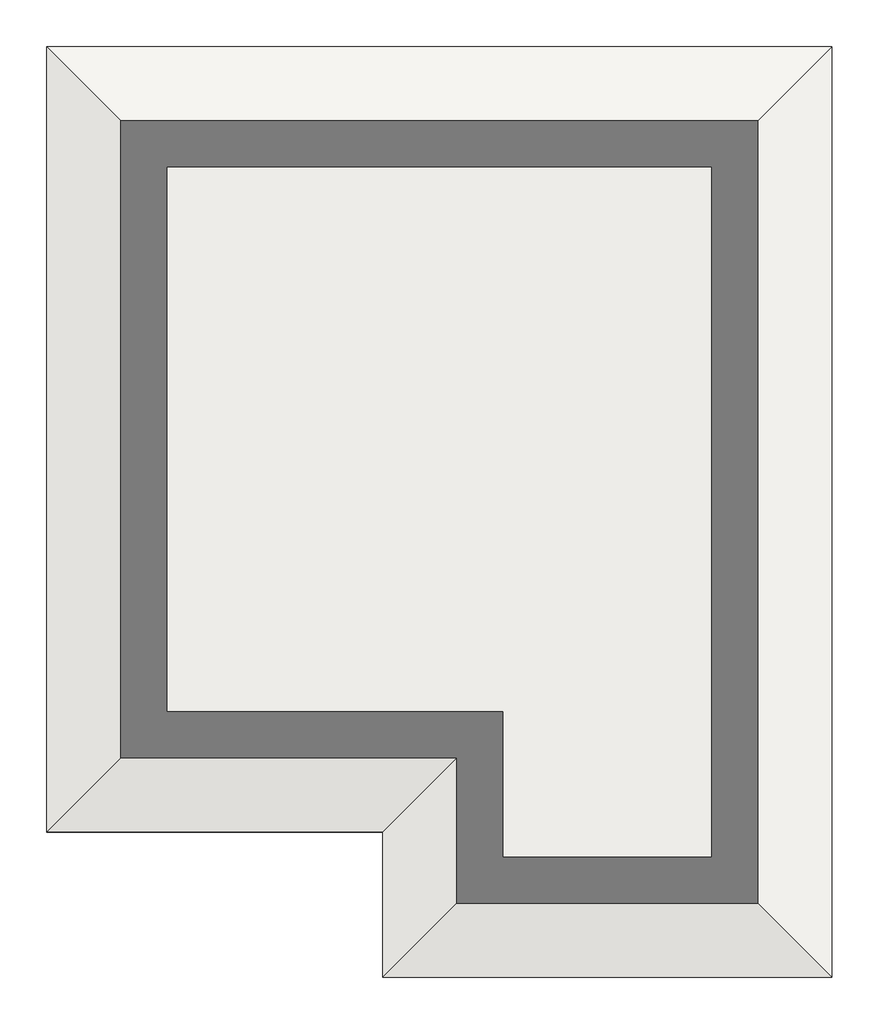
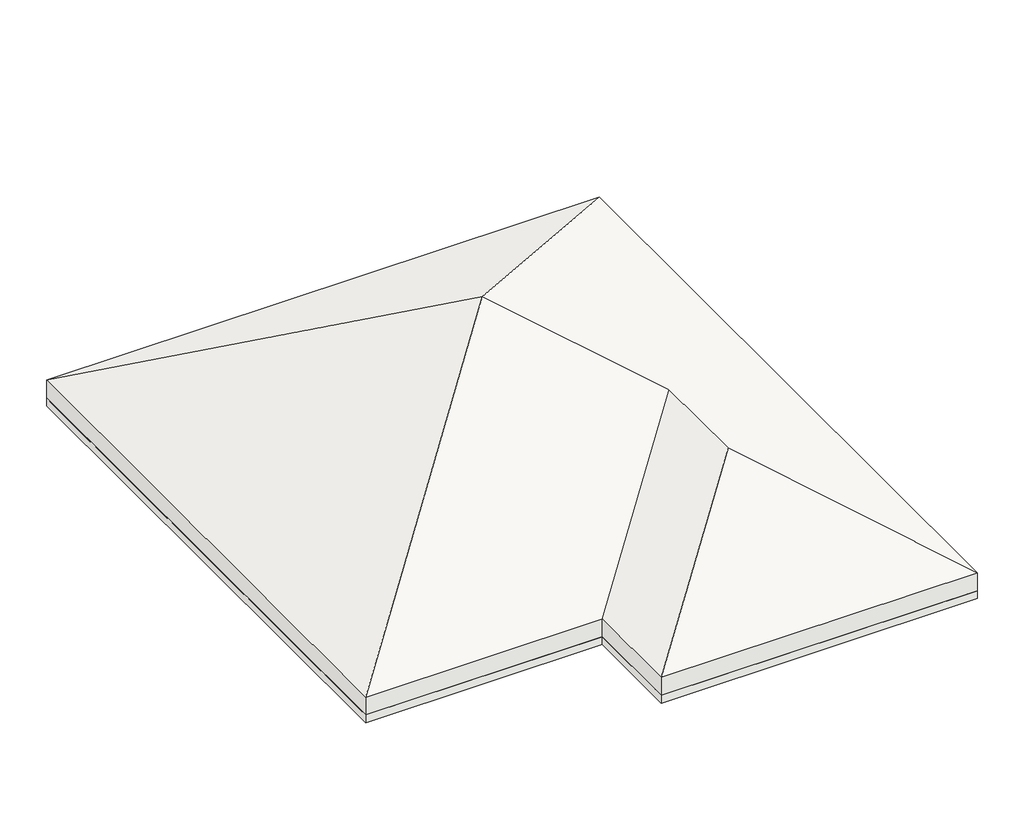
# One storey: 15 beams, 6 walls, 1 roof, 1 slab.
"""IFC4 building model written with IfcOpenShell, lengths in millimetres."""

import ifcopenshell
import ifcopenshell.guid

model = None  # the IFC model being written
_history = None  # IfcOwnerHistory: only IFC2X3 demands one
_inside = {}  # id of a spatial element -> (the spatial element, [elements in it])
_under = {}  # id of a project, library or spatial element -> (it, [spatial elements below it])
_declared = {}  # id of a project -> (the project, [libraries it declares])
_typed = {}  # id of a type object -> (the type object, [elements of that type])
_made_of = {}  # id of a material, layer set ... -> (it, [elements and type objects made of it])


def new_model(schema):
    """Start an empty IFC model of exactly this schema.

    Asked for "IFC4X3", IfcOpenShell would pick the latest addendum, in which some entities
    have other attributes; the version numbers below select the first issue.
    IFC2X3 requires an IfcOwnerHistory on every rooted entity: one is made here for all.
    """
    global model, _history
    if schema == "IFC4X3":
        model = ifcopenshell.file(schema_version=(4, 3, 0, 0))
    else:
        model = ifcopenshell.file(schema=schema)
    _inside.clear()
    _under.clear()
    _declared.clear()
    _typed.clear()
    _made_of.clear()
    _history = None
    if model.schema == "IFC2X3":
        org = make("IfcOrganization", Name="unknown")
        user = make(
            "IfcPersonAndOrganization",
            ThePerson=make("IfcPerson", FamilyName="unknown"),
            TheOrganization=org,
        )
        app = make(
            "IfcApplication",
            ApplicationDeveloper=org,
            Version="unknown",
            ApplicationFullName="unknown",
            ApplicationIdentifier="unknown",
        )
        _history = make(
            "IfcOwnerHistory",
            OwningUser=user,
            OwningApplication=app,
            ChangeAction="ADDED",
            CreationDate=0,
        )
    return model


def make(cls, **values):
    """One entity of the class cls with the attributes given. An attribute that is None is left unset."""
    return model.create_entity(
        cls, **{name: value for name, value in values.items() if value is not None}
    )


def rooted(cls, **values):
    """An entity with a GlobalId (a new one), such as an element, a storey or a relation."""
    return make(cls, GlobalId=ifcopenshell.guid.new(), OwnerHistory=_history, **values)


def si_unit(unit_type, name, prefix=None):
    """IfcSIUnit, for example si_unit("LENGTHUNIT", "METRE", prefix="MILLI")."""
    return make("IfcSIUnit", UnitType=unit_type, Prefix=prefix, Name=name)


def assignment(units):
    """IfcUnitAssignment: the units of a project."""
    return None if units is None else make("IfcUnitAssignment", Units=units)


def point(xyz):
    """IfcCartesianPoint."""
    return None if xyz is None else make("IfcCartesianPoint", Coordinates=xyz)


def direction(xyz):
    """IfcDirection."""
    return None if xyz is None else make("IfcDirection", DirectionRatios=xyz)


def frame(location, z_axis=None, x_axis=None):
    """IfcAxis2Placement3D, a coordinate frame: its origin and axes. An axis left out is left unset."""
    return make(
        "IfcAxis2Placement3D",
        Location=point(location),
        Axis=direction(z_axis),
        RefDirection=direction(x_axis),
    )


def origin():
    """The frame at (0, 0, 0) with its axes left unset."""
    return frame((0.0, 0.0, 0.0))


def place(relative_to, where):
    """IfcLocalPlacement: puts the frame where relative to a parent placement (None: the world)."""
    return make(
        "IfcLocalPlacement", PlacementRelTo=relative_to, RelativePlacement=where
    )


def context(
    kind, dimensions, precision=None, world=None, true_north=None, identifier=None
):
    """IfcGeometricRepresentationContext, for example the 3D "Model" context."""
    return make(
        "IfcGeometricRepresentationContext",
        ContextIdentifier=identifier,
        ContextType=kind,
        CoordinateSpaceDimension=dimensions,
        Precision=precision,
        WorldCoordinateSystem=world,
        TrueNorth=true_north,
    )


def project(units=None, contexts=None):
    """IfcProject with its units and contexts."""
    return rooted(
        "IfcProject",
        Name="project",
        RepresentationContexts=contexts,
        UnitsInContext=assignment(units),
    )


def spatial(cls, under=None, at=None, **own):
    """A site, building, storey or space (cls), placed at a placement, below another one or the project."""
    s = rooted(cls, ObjectPlacement=at, **own)
    if under is not None:
        _under.setdefault(under.id(), (under, []))[1].append(s)
    return s


def polyline(points):
    """IfcPolyline through the points."""
    return make("IfcPolyline", Points=[point(p) for p in points])


def outline(outer, holes=None, kind="AREA"):
    """IfcArbitraryClosedProfileDef: a profile drawn as a closed curve; with holes, ...WithVoids."""
    if holes is None:
        return make("IfcArbitraryClosedProfileDef", ProfileType=kind, OuterCurve=outer)
    return make(
        "IfcArbitraryProfileDefWithVoids",
        ProfileType=kind,
        OuterCurve=outer,
        InnerCurves=holes,
    )


def extrude(swept, where, along, depth):
    """IfcExtrudedAreaSolid: the profile swept, set in the frame where, extruded along a direction by depth."""
    return make(
        "IfcExtrudedAreaSolid",
        SweptArea=swept,
        Position=where,
        ExtrudedDirection=direction(along),
        Depth=depth,
    )


def faces_of(points, faces, orient=None, outer=None):
    """IfcFace entities. A face is a list of loops; a loop is a list of indices into points, from 0.

    orient and outer hold one flag for each loop. By default every Orientation is true, the
    first loop of a face is its IfcFaceOuterBound and the others are IfcFaceBound.
    """
    made = []
    for i, loops in enumerate(faces):
        bounds = []
        for j, loop in enumerate(loops):
            is_outer = j == 0 if outer is None else outer[i][j]
            bounds.append(
                make(
                    "IfcFaceOuterBound" if is_outer else "IfcFaceBound",
                    Bound=make("IfcPolyLoop", Polygon=[points[k] for k in loop]),
                    Orientation=True if orient is None else orient[i][j],
                )
            )
        made.append(make("IfcFace", Bounds=bounds))
    return made


def faceted_brep(points, faces, orient=None, outer=None, voids=None):
    """IfcFacetedBrep: a solid bounded by flat faces; with voids (closed shells), ...WithVoids."""
    shared = [point(p) for p in points]
    hull = make("IfcClosedShell", CfsFaces=faces_of(shared, faces, orient, outer))
    if voids is None:
        return make("IfcFacetedBrep", Outer=hull)
    return make(
        "IfcFacetedBrepWithVoids",
        Outer=hull,
        Voids=[
            make(cls, CfsFaces=faces_of(shared, fs, o, b)) for cls, fs, o, b in voids
        ],
    )


def shape(context_of_items, identifier, shape_type, items):
    """IfcShapeRepresentation: the items that make up one representation, for example the "Body"."""
    return make(
        "IfcShapeRepresentation",
        ContextOfItems=context_of_items,
        RepresentationIdentifier=identifier,
        RepresentationType=shape_type,
        Items=items,
    )


def made_of(thing, what):
    """Note that an element or type object is made of a material, layer set ...; save() writes the relation."""
    if what is not None:
        _made_of.setdefault(what.id(), (what, []))[1].append(thing)
    return thing


def element(
    cls,
    number,
    at=None,
    inside=None,
    cuts=None,
    type_object=None,
    material=None,
    context=None,
    identifier="Body",
    shape_type=None,
    held_by="IfcProductDefinitionShape",
    body=None,
    shapes=None,
    **own,
):
    """One element of the class cls, such as IfcWall. Its Tag is "e" and its number.

    at: its placement. inside: the storey or other place that contains it. cuts: it is an
    opening in that element (IfcRelVoidsElement). A single representation is given by context,
    identifier, shape_type and body (its items); several are given by shapes. held_by: the class
    of the entity that holds the representations. save() writes the other relations.
    """
    e = rooted(cls, Tag="e%d" % number, ObjectPlacement=at, **own)
    if body is not None:
        shapes = [shape(context, identifier, shape_type, body)]
    if shapes is not None:
        e.Representation = make(held_by, Representations=shapes)
    if inside is not None:
        _inside.setdefault(inside.id(), (inside, []))[1].append(e)
    if cuts is not None:
        rooted(
            "IfcRelVoidsElement", RelatingBuildingElement=cuts, RelatedOpeningElement=e
        )
    if type_object is not None:
        _typed.setdefault(type_object.id(), (type_object, []))[1].append(e)
    return made_of(e, material)


def aggregate(whole, parts):
    """IfcRelAggregates: a whole, such as a stair, and the parts it consists of."""
    return rooted("IfcRelAggregates", RelatingObject=whole, RelatedObjects=parts)


def save(model, path):
    """Write the relations noted so far, then the file.

    IfcRelAggregates (storeys below a building ...), IfcRelContainedInSpatialStructure (elements
    in a storey), IfcRelDefinesByType, IfcRelAssociatesMaterial and IfcRelDeclares: one each for
    every whole, place, type object, material and project.
    """
    for whole, parts in _under.values():
        aggregate(whole, parts)
    for where, things in _inside.values():
        rooted(
            "IfcRelContainedInSpatialStructure",
            RelatedElements=things,
            RelatingStructure=where,
        )
    for kind, things in _typed.values():
        rooted("IfcRelDefinesByType", RelatedObjects=things, RelatingType=kind)
    for what, things in _made_of.values():
        rooted("IfcRelAssociatesMaterial", RelatedObjects=things, RelatingMaterial=what)
    for by, libraries in _declared.values():
        rooted("IfcRelDeclares", RelatingContext=by, RelatedDefinitions=libraries)
    model.write(path)


model = new_model("IFC4")

# Units and contexts
model_context = context("Model", 3, world=origin())
ifc_project = project(units=[si_unit("LENGTHUNIT", "METRE", prefix="MILLI")], contexts=[model_context])

# Site, building, storey
site = spatial("IfcSite", under=ifc_project)
building = spatial("IfcBuilding", under=site)
storey = spatial("IfcBuildingStorey", under=building, Name="02-Çatı Katı", Elevation=100780.0)

# Beams
placement = place(None, origin())
element("IfcBeam", 1, ObjectType="M_Concrete-Rectangular Beam : 45x60cm Kiriş", at=placement, inside=storey, context=model_context, shape_type="SweptSolid", body=[
    extrude(outline(polyline([(5700.0, 14550.0), (450.0, 14550.0), (450.0, 15000.0), (5700.0, 15000.0), (5700.0, 14550.0)])), frame((0.0, 0.0, 100180.0), z_axis=(0.0, 0.0, 1.0), x_axis=(1.0, 0.0, 0.0)), (0.0, 0.0, 1.0), 400.0),
])
element("IfcBeam", 2, ObjectType="M_Concrete-Rectangular Beam : 45x60cm Kiriş", at=placement, inside=storey, context=model_context, shape_type="SweptSolid", body=[
    extrude(outline(polyline([(0.0, 3100.0), (0.0, 8200.0), (450.0, 8200.0), (450.0, 3100.0), (0.0, 3100.0)])), frame((0.0, 0.0, 100180.0), z_axis=(0.0, 0.0, 1.0), x_axis=(1.0, 0.0, 0.0)), (0.0, 0.0, 1.0), 400.0),
])
element("IfcBeam", 3, ObjectType="M_Concrete-Rectangular Beam : 45x60cm Kiriş", at=placement, inside=storey, context=model_context, shape_type="SweptSolid", body=[
    extrude(outline(polyline([(5700.0, 2500.0), (450.0, 2500.0), (450.0, 2950.0), (5700.0, 2950.0), (5700.0, 2500.0)])), frame((0.0, 0.0, 100180.0), z_axis=(0.0, 0.0, 1.0), x_axis=(1.0, 0.0, 0.0)), (0.0, 0.0, 1.0), 400.0),
])
element("IfcBeam", 4, ObjectType="M_Concrete-Rectangular Beam : 45x60cm Kiriş", at=placement, inside=storey, context=model_context, shape_type="SweptSolid", body=[
    extrude(outline(polyline([(12050.0, 2500.0), (6300.0, 2500.0), (6300.0, 2950.0), (12050.0, 2950.0), (12050.0, 2500.0)])), frame((0.0, 0.0, 100180.0), z_axis=(0.0, 0.0, 1.0), x_axis=(1.0, 0.0, 0.0)), (0.0, 0.0, 1.0), 400.0),
])
element("IfcBeam", 5, ObjectType="M_Concrete-Rectangular Beam : 45x60cm Kiriş", at=placement, inside=storey, context=model_context, shape_type="SweptSolid", body=[
    extrude(outline(polyline([(12500.0, 8200.0), (12500.0, 3100.0), (12050.0, 3100.0), (12050.0, 8200.0), (12500.0, 8200.0)])), frame((0.0, 0.0, 100180.0), z_axis=(0.0, 0.0, 1.0), x_axis=(1.0, 0.0, 0.0)), (0.0, 0.0, 1.0), 400.0),
])
element("IfcBeam", 6, ObjectType="M_Concrete-Rectangular Beam : 45x60cm Kiriş", at=placement, inside=storey, context=model_context, shape_type="SweptSolid", body=[
    extrude(outline(polyline([(0.0, 8800.0), (0.0, 14400.0), (450.0, 14400.0), (450.0, 8800.0), (0.0, 8800.0)])), frame((0.0, 0.0, 100180.0), z_axis=(0.0, 0.0, 1.0), x_axis=(1.0, 0.0, 0.0)), (0.0, 0.0, 1.0), 400.0),
])
element("IfcBeam", 7, ObjectType="M_Concrete-Rectangular Beam : 45x60cm Kiriş", at=placement, inside=storey, context=model_context, shape_type="SweptSolid", body=[
    extrude(outline(polyline([(5775.0, 8800.0), (5775.0, 14550.0), (6225.0, 14550.0), (6225.0, 8800.0), (5775.0, 8800.0)])), frame((0.0, 0.0, 100180.0), z_axis=(0.0, 0.0, 1.0), x_axis=(1.0, 0.0, 0.0)), (0.0, 0.0, 1.0), 400.0),
])
element("IfcBeam", 8, ObjectType="M_Concrete-Rectangular Beam : 30x60cm Kiriş", at=placement, inside=storey, context=model_context, shape_type="SweptSolid", body=[
    extrude(outline(polyline([(9850.0, 15000.0), (9850.0, 14700.0), (6300.0, 14700.0), (6300.0, 15000.0), (9850.0, 15000.0)])), frame((0.0, 0.0, 100180.0), z_axis=(0.0, 0.0, 1.0), x_axis=(1.0, 0.0, 0.0)), (0.0, 0.0, 1.0), 400.0),
])
element("IfcBeam", 9, ObjectType="M_Concrete-Rectangular Beam : 30x60cm Kiriş", at=placement, inside=storey, context=model_context, shape_type="SweptSolid", body=[
    extrude(outline(polyline([(12200.0, 10850.0), (12500.0, 10850.0), (12500.0, 8800.0), (12200.0, 8800.0), (12200.0, 10850.0)])), frame((0.0, 0.0, 100180.0), z_axis=(0.0, 0.0, 1.0), x_axis=(1.0, 0.0, 0.0)), (0.0, 0.0, 1.0), 400.0),
])
element("IfcBeam", 10, ObjectType="M_Concrete-Rectangular Beam : 45x60cm Kiriş", at=placement, inside=storey, context=model_context, shape_type="SweptSolid", body=[
    extrude(outline(polyline([(5775.0, 2950.0), (5775.0, 8200.0), (6225.0, 8200.0), (6225.0, 2950.0), (5775.0, 2950.0)])), frame((0.0, 0.0, 100180.0), z_axis=(0.0, 0.0, 1.0), x_axis=(1.0, 0.0, 0.0)), (0.0, 0.0, 1.0), 400.0),
])
element("IfcBeam", 11, ObjectType="M_Concrete-Rectangular Beam : 45x60cm Kiriş", at=placement, inside=storey, context=model_context, shape_type="SweptSolid", body=[
    extrude(outline(polyline([(5775.0, 8275.0), (450.0, 8275.0), (450.0, 8725.0), (5775.0, 8725.0), (5775.0, 8275.0)])), frame((0.0, 0.0, 100180.0), z_axis=(0.0, 0.0, 1.0), x_axis=(1.0, 0.0, 0.0)), (0.0, 0.0, 1.0), 400.0),
])
element("IfcBeam", 12, ObjectType="M_Concrete-Rectangular Beam : 45x60cm Kiriş", at=placement, inside=storey, context=model_context, shape_type="SweptSolid", body=[
    extrude(outline(polyline([(12050.0, 8275.0), (6225.0, 8275.0), (6225.0, 8725.0), (12050.0, 8725.0), (12050.0, 8275.0)])), frame((0.0, 0.0, 100180.0), z_axis=(0.0, 0.0, 1.0), x_axis=(1.0, 0.0, 0.0)), (0.0, 0.0, 1.0), 400.0),
])
element("IfcBeam", 13, ObjectType="M_Concrete-Rectangular Beam : 45x60cm Kiriş", at=placement, inside=storey, context=model_context, shape_type="Brep", body=[
    faceted_brep([(5775.0, 2500.0, 100180.0), (5775.0, 400.0, 100180.0), (5775.0, 400.0, 100580.0), (5775.0, 2500.0, 100580.0), (6225.0, 2500.0, 100180.0), (6225.0, 450.0, 100180.0), (6225.0, 0.0, 100180.0), (6175.0, 0.0, 100180.0), (6175.0, 400.0, 100180.0), (6225.0, 2500.0, 100580.0), (6225.0, 450.0, 100580.0), (6225.0, 0.0, 100580.0), (6175.0, 0.0, 100580.0), (6175.0, 400.0, 100580.0)], [[[0, 1, 2, 3]], [[0, 4, 5, 6, 7, 8, 1]], [[6, 5, 4, 9, 10, 11]], [[4, 0, 3, 9]], [[8, 7, 12, 13]], [[1, 8, 13, 2]], [[7, 6, 11, 12]], [[3, 2, 13, 12, 11, 10, 9]]]),
])
element("IfcBeam", 14, ObjectType="M_Concrete-Rectangular Beam : 45x60cm Kiriş", at=placement, inside=storey, context=model_context, shape_type="Brep", body=[
    faceted_brep([(6225.0, 0.0, 100180.0), (12100.0, 0.0, 100180.0), (12100.0, 0.0, 100580.0), (6225.0, 0.0, 100580.0), (6225.0, 450.0, 100180.0), (12050.0, 450.0, 100180.0), (12500.0, 450.0, 100180.0), (12500.0, 400.0, 100180.0), (12100.0, 400.0, 100180.0), (6225.0, 450.0, 100580.0), (12050.0, 450.0, 100580.0), (12500.0, 450.0, 100580.0), (12100.0, 400.0, 100580.0), (12500.0, 400.0, 100580.0)], [[[0, 1, 2, 3]], [[0, 4, 5, 6, 7, 8, 1]], [[6, 5, 4, 9, 10, 11]], [[4, 0, 3, 9]], [[1, 8, 12, 2]], [[8, 7, 13, 12]], [[7, 6, 11, 13]], [[3, 2, 12, 13, 11, 10, 9]]]),
])
element("IfcBeam", 15, ObjectType="M_Concrete-Rectangular Beam : 45x60cm Kiriş", at=placement, inside=storey, context=model_context, shape_type="SweptSolid", body=[
    extrude(outline(polyline([(12050.0, 2500.0), (12500.0, 2500.0), (12500.0, 450.0), (12050.0, 450.0), (12050.0, 2500.0)])), frame((0.0, 0.0, 100180.0), z_axis=(0.0, 0.0, 1.0), x_axis=(1.0, 0.0, 0.0)), (0.0, 0.0, 1.0), 400.0),
])

# Roof
element("IfcRoof", 16, ObjectType="Generic - 400mm", at=placement, inside=storey, context=model_context, shape_type="Brep", body=[
    faceted_brep([(-500.0, 2000.0, 100780.0), (-500.0, 15500.0, 100780.0), (6250.0, 8750.0, 104677.114317), (9137.5, 5862.5, 103010.0154147), (5275.0, 2000.0, 100780.0), (5275.0, -500.0, 100780.0), (9137.5, 3362.5, 103010.0154147), (13000.0, -500.0, 100780.0), (13000.0, 15500.0, 100780.0), (-500.0, 2000.0, 101241.8802154), (6250.0, 8750.0, 105138.9945324), (-500.0, 15500.0, 101241.8802154), (5275.0, 2000.0, 101241.8802154), (9137.5, 5862.5, 103471.8956301), (5275.0, -500.0, 101241.8802154), (13000.0, -500.0, 101241.8802154), (9137.5, 3362.5, 103471.8956301), (13000.0, 15500.0, 101241.8802154)], [[[0, 1, 2]], [[0, 2, 3, 4]], [[5, 6, 7]], [[8, 2, 1]], [[7, 6, 3, 2, 8]], [[5, 4, 3, 6]], [[9, 10, 11]], [[9, 12, 13, 10]], [[14, 15, 16]], [[17, 11, 10]], [[15, 17, 10, 13, 16]], [[12, 14, 16, 13]], [[4, 12, 9, 0]], [[5, 14, 12, 4]], [[7, 15, 14, 5]], [[8, 17, 15, 7]], [[1, 11, 17, 8]], [[0, 9, 11, 1]]]),
])

# Slab
element("IfcSlab", 17, ObjectType="20 cm döşeme", at=placement, inside=storey, context=model_context, shape_type="SweptSolid", body=[
    extrude(outline(polyline([(-500.0, 15500.0), (13000.0, 15500.0), (13000.0, -500.0), (5275.0, -500.0), (5275.0, 2000.0), (-500.0, 2000.0), (-500.0, 15500.0)])), frame((0.0, 0.0, 100580.0), z_axis=(0.0, 0.0, 1.0), x_axis=(1.0, 0.0, 0.0)), (0.0, 0.0, 1.0), 200.0),
])

# Walls
element("IfcWall", 18, ObjectType="25cm Perde Duvar", at=placement, inside=storey, context=model_context, shape_type="Brep", body=[
    faceted_brep([(-500.0, 15250.0, 100780.0), (-250.0, 15250.0, 100780.0), (12750.0, 15250.0, 100780.0), (13000.0, 15250.0, 100780.0), (12750.0, 15250.0, 100924.3375673), (-250.0, 15250.0, 100924.3375673), (-500.0, 15500.0, 100780.0), (13000.0, 15500.0, 100780.0)], [[[0, 1, 2, 3, 4, 5]], [[3, 2, 1, 0, 6, 7]], [[0, 5, 6]], [[5, 4, 7, 6]], [[4, 3, 7]]]),
])
element("IfcWall", 19, ObjectType="25cm Perde Duvar", at=placement, inside=storey, context=model_context, shape_type="Brep", body=[
    faceted_brep([(12750.0, 15250.0, 100780.0), (12750.0, -250.0, 100780.0), (12750.0, -500.0, 100780.0), (12750.0, -250.0, 100924.3375673), (12750.0, 15250.0, 100924.3375673), (13000.0, 15250.0, 100780.0), (13000.0, -500.0, 100780.0)], [[[0, 1, 2, 3, 4]], [[2, 1, 0, 5, 6]], [[0, 4, 5]], [[4, 3, 6, 5]], [[3, 2, 6]]]),
])
element("IfcWall", 20, ObjectType="25cm Perde Duvar", at=placement, inside=storey, context=model_context, shape_type="Brep", body=[
    faceted_brep([(12750.0, -250.0, 100780.0), (5525.0, -250.0, 100780.0), (5275.0, -250.0, 100780.0), (5525.0, -250.0, 100924.3375673), (12750.0, -250.0, 100924.3375673), (12750.0, -500.0, 100780.0), (5275.0, -500.0, 100780.0)], [[[0, 1, 2, 3, 4]], [[2, 1, 0, 5, 6]], [[0, 4, 5]], [[4, 3, 6, 5]], [[3, 2, 6]]]),
])
element("IfcWall", 21, ObjectType="25cm Perde Duvar", at=placement, inside=storey, context=model_context, shape_type="SweptSolid", body=[
    extrude(outline(polyline([(100780.0, 5275.0), (100780.0, 5525.0), (100924.3375673, 5525.0), (100780.0, 5275.0)])), frame((0.0, -250.0, 0.0), z_axis=(0.0, 1.0, 0.0), x_axis=(0.0, 0.0, 1.0)), (0.0, 0.0, 1.0), 2500.0),
])
element("IfcWall", 22, ObjectType="25cm Perde Duvar", at=placement, inside=storey, context=model_context, shape_type="Brep", body=[
    faceted_brep([(5275.0, 2250.0, 100780.0), (-250.0, 2250.0, 100780.0), (-500.0, 2250.0, 100780.0), (-250.0, 2250.0, 100924.3375673), (5275.0, 2250.0, 100924.3375673), (5275.0, 2000.0, 100780.0), (-500.0, 2000.0, 100780.0)], [[[0, 1, 2, 3, 4]], [[2, 1, 0, 5, 6]], [[0, 4, 5]], [[4, 3, 6, 5]], [[3, 2, 6]]]),
])
element("IfcWall", 23, ObjectType="25cm Perde Duvar", at=placement, inside=storey, context=model_context, shape_type="SweptSolid", body=[
    extrude(outline(polyline([(100780.0, -250.0), (100924.3375673, -250.0), (100780.0, -500.0), (100780.0, -250.0)])), frame((0.0, 2250.0, 0.0), z_axis=(0.0, 1.0, 0.0), x_axis=(0.0, 0.0, 1.0)), (0.0, 0.0, 1.0), 13000.0),
])

save(model, "model.ifc")

# Revit data of these elements
# Type "M_Concrete-Rectangular Beam : 45x60cm Kiriş"
#   Length [instance default] = 152.40 cm
#   b = 45.00 cm
#   h = 60.00 cm
#   Structural Material [instance default] = Concrete, Cast-in-Place gray
#   Assembly Code = ""
# Type "M_Concrete-Rectangular Beam : 30x60cm Kiriş"
#   Length [instance default] = 152.40 cm
#   b = 30.00 cm
#   h = 60.00 cm
#   Structural Material [instance default] = Concrete, Cast-in-Place gray
#   Assembly Code = ""
# Type "Generic - 400mm"
#   Layers, outside or top first: 40.00 cm no material (function 1)
# Type "20 cm döşeme"
#   Function = 0
#   Layers, outside or top first: 20.00 cm "Concrete, Cast In Situ" (function 1)
# Type "25cm Perde Duvar"
#   Layers, outside or top first: 25.00 cm "Concrete, Cast In Situ" (function 1)
# Elements 1, 2, 3, 4, 5, 6, 7, 10, 11, 12, 13, 14, 15 (IfcBeam, "M_Concrete-Rectangular Beam : 45x60cm Kiriş")
#   Comments = ""
#   Structural Material = Concrete, Cast-in-Place gray
#   Phase Created = New Construction
#   Materials on its faces: "Concrete, Cast-in-Place gray"
# Elements 8, 9 (IfcBeam, "M_Concrete-Rectangular Beam : 30x60cm Kiriş")
#   Comments = ""
#   Structural Material = Concrete, Cast-in-Place gray
#   Phase Created = New Construction
#   Materials on its faces: "Concrete, Cast-in-Place gray"
# Element 16 (IfcRoof, "Generic - 400mm")
#   built-in parameter 1001705 = 344.944 (stored number, unit not read)
#   built-in parameter 1001710 = 33615
#   Phase Created = New Construction
#   Materials on its faces: "Default Roof"
# Element 17 (IfcSlab, "20 cm döşeme")
#   Height Offset From Level = 0.00 cm
#   built-in parameter 1001954 = 1
#   Phase Created = New Construction
#   Materials on its faces: "Concrete, Cast In Situ"
# Elements 18, 19, 20, 21, 22, 23 (IfcWall, "25cm Perde Duvar")
#   Comments = ""
#   Top Offset = 0.00 cm
#   Base Offset = 0.00 cm
#   Unconnected Height = 60.00 cm
#   wall height = 60.00 cm
#   Phase Created = New Construction
#   Base Constraint = 02-Çatı Katı
#   Materials on its faces: "Concrete, Cast In Situ"
# Materials
#   "Concrete, Cast-in-Place gray": class "Concrete", colour RGB 192 192 192, transparency 0, Description = "Cast-in-place concrete", Cost = 0
#   "Concrete, Cast In Situ": class "Concrete", colour RGB 192 192 192, transparency 0, Description = "physical material", Cost = 0
#   "Default Roof": class "Miscellaneous", colour RGB 0 127 0, transparency 0
